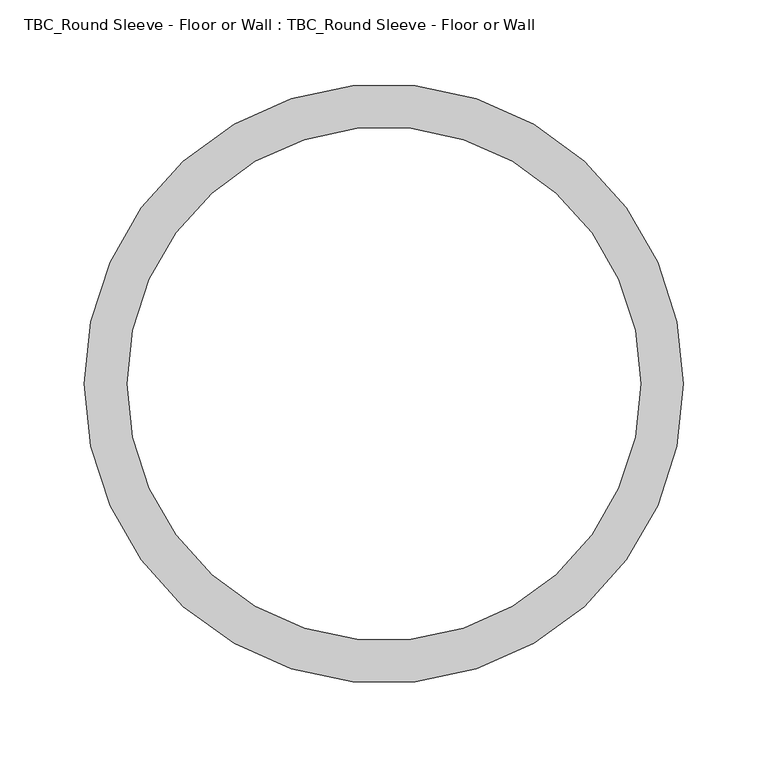
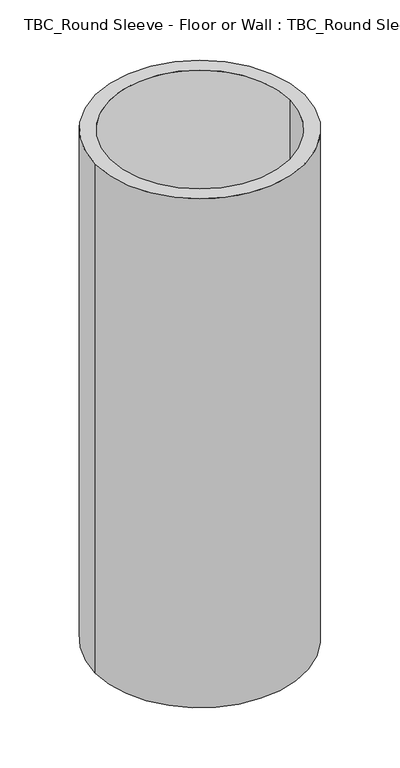
"""IFC4 building model written with IfcOpenShell, lengths in millimetres: proxy geometry, TBC_Round Sleeve - Floor or Wall : TBC_Round Sleeve - Floor or Wall."""

from ifc_helpers import new_model, si_unit, point, frame, origin, origin_2d, place, context, project, spatial, circle_curve, trimmed, segment, composite_curve, outline, extrude, source, transform, mapped, element, save


def tbc_round_sleeve_floor_or_wall_tbc_round_sleeve_floor_or_7fc3faad(model_context):
    return source(origin(), model_context, "Body", "SweptSolid", [
        extrude(outline(composite_curve([segment(trimmed(circle_curve(origin_2d(), 177.8), [point((-177.8, 0.0))], [point((177.8, 0.0))], False, "CARTESIAN"), True, "CONTINUOUS"), segment(trimmed(circle_curve(origin_2d(), 177.8), [point((177.8, 0.0))], [point((-177.8, 0.0))], False, "CARTESIAN"), True, "CONTINUOUS")], self_intersect=False), holes=[composite_curve([segment(trimmed(circle_curve(origin_2d(), 152.4), [point((-152.4, 0.0))], [point((152.4, 0.0))], True, "CARTESIAN"), True, "CONTINUOUS"), segment(trimmed(circle_curve(origin_2d(), 152.4), [point((152.4, 0.0))], [point((-152.4, 0.0))], True, "CARTESIAN"), True, "CONTINUOUS")], self_intersect=False)]), frame((0.0, 0.0, -914.4), z_axis=(0.0, 0.0, 1.0), x_axis=(1.0, 0.0, 0.0)), (0.0, 0.0, 1.0), 914.4),
    ])


if __name__ == "__main__":
    model = new_model("IFC4")
    model_context = context("Model", 3, world=origin())
    ifc_project = project(units=[si_unit("LENGTHUNIT", "METRE", prefix="MILLI")], contexts=[model_context])
    site = spatial("IfcSite", under=ifc_project)
    building = spatial("IfcBuilding", under=site)
    placement = place(None, origin())
    tbc_round_sleeve_floor_or_wall_tbc_round_sleeve_floor_or_shape = tbc_round_sleeve_floor_or_wall_tbc_round_sleeve_floor_or_7fc3faad(model_context)
    element("IfcBuildingElementProxy", 1, Name="TBC_Round Sleeve - Floor or Wall : TBC_Round Sleeve - Floor or Wall", ObjectType="TBC_Round Sleeve - Floor or Wall : TBC_Round Sleeve - Floor or Wall", at=placement, inside=building, context=model_context, shape_type="MappedRepresentation", body=[
        mapped(tbc_round_sleeve_floor_or_wall_tbc_round_sleeve_floor_or_shape, transform((0.0, 0.0, 0.0), x_axis=(1.0, 0.0, 0.0), y_axis=(0.0, 1.0, 0.0), z_axis=(0.0, 0.0, 1.0))),
    ])
    save(model, "model.ifc")

# Revit data of these elements
# Project information
#   Project Issue Date = "Issue Date"
#   Project Status = "Project Status"
#   Client Name = "Owner"
#   Project Address = "Enter address here"
#   Project Name = "Project Name"
#   Project Number = "Project Number"
# Type "TBC_Round Sleeve - Floor or Wall : TBC_Round Sleeve - Floor or Wall"
#   Tag Dimension [instance default] = ""
#   MEP Type [instance default] = ""
#   MEP Element [instance default] = ""
#   MEP Category [instance default] = ""
#   Host Element Type [instance default] = ""
#   Host Element Id [instance default] = ""
#   Host Element Category [instance default] = ""
#   Control Line Y [instance default] = ""
#   Control Line X [instance default] = ""
#   Sleeve Radius [instance default] = 1' - 0"
#   Sleeve Edge [instance default] = 1' - 2"
#   Sleeve Depth [instance default] = 3' - 0"
#   Distance Y [instance default] = 0' - 0"
#   Distance X [instance default] = 0' - 0"
#   Default Elevation = 0
